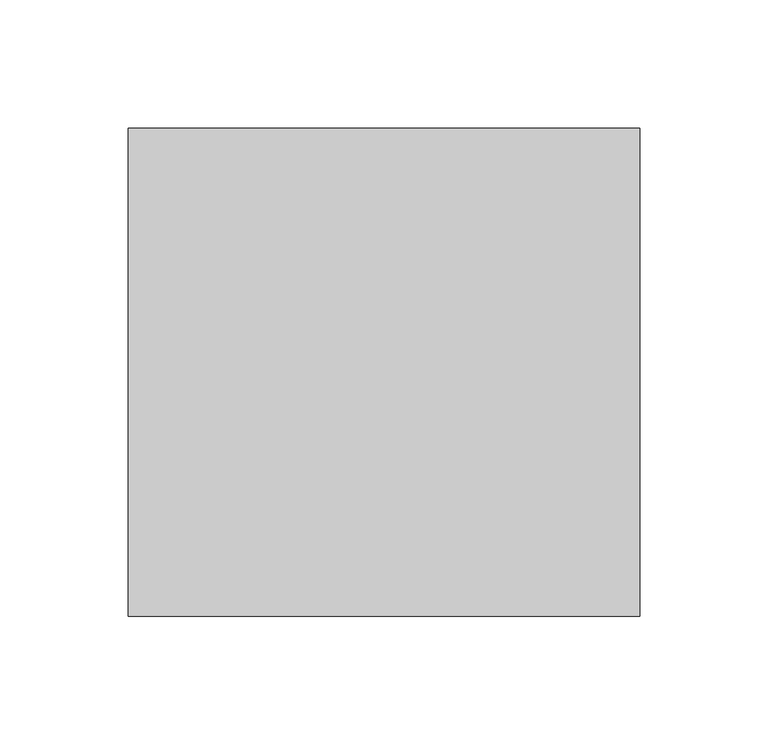
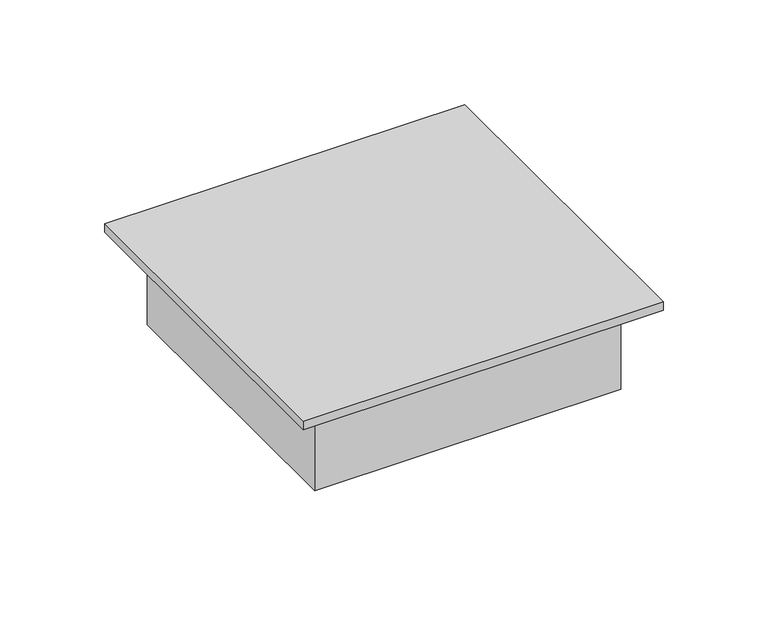
"""IFC4 building model written with IfcOpenShell, lengths in millimetres: proxy geometry, CAIXA VERTICE V7 : QD Amanco Passagem Pequena."""

from ifc_helpers import new_model, si_unit, origin, origin_with_axes, place, context, project, spatial, polyline, outline, extrude, faceted_brep, source, transform, mapped, element, save


def electrical_fixtures_13f3b859(model_context):
    return source(origin(), model_context, "Body", "SolidModel", [
        faceted_brep([(82.5, 1022.0, -48.0), (82.5, 1178.0, -48.0), (-82.5, 1178.0, -48.0), (-82.5, 1022.0, -48.0), (84.5, 1180.0, -50.0), (84.5, 1020.0, -50.0), (-84.5, 1020.0, -50.0), (-84.5, 1180.0, -50.0), (-84.5, 1180.0, 0.0), (84.5, 1180.0, 0.0), (-84.5, 1020.0, 0.0), (84.5, 1020.0, 0.0), (82.5, 1178.0, 0.0), (82.5, 1022.0, 0.0), (-82.5, 1022.0, 0.0), (-82.5, 1178.0, 0.0)], [[[0, 1, 2, 3]], [[4, 5, 6, 7]], [[4, 7, 8, 9]], [[8, 7, 6, 10]], [[10, 6, 5, 11]], [[11, 5, 4, 9]], [[9, 8, 10, 11], [12, 13, 14, 15]], [[13, 12, 1, 0]], [[14, 13, 0, 3]], [[15, 14, 3, 2]], [[12, 15, 2, 1]]]),
        extrude(outline(polyline([(99.5, 1195.0), (99.5, 1005.0), (-99.5, 1005.0), (-99.5, 1195.0), (99.5, 1195.0)])), origin_with_axes(), (0.0, 0.0, 1.0), 5.0),
    ])


if __name__ == "__main__":
    model = new_model("IFC4")
    model_context = context("Model", 3, world=origin())
    ifc_project = project(units=[si_unit("LENGTHUNIT", "METRE", prefix="MILLI")], contexts=[model_context])
    site = spatial("IfcSite", under=ifc_project)
    building = spatial("IfcBuilding", under=site)
    placement = place(None, origin())
    electrical_fixtures_shape = electrical_fixtures_13f3b859(model_context)
    element("IfcBuildingElementProxy", 1, Name="CAIXA VERTICE V7 : QD Amanco Passagem Pequena", ObjectType="CAIXA VERTICE V7 : QD Amanco Passagem Pequena", at=placement, inside=building, context=model_context, shape_type="MappedRepresentation", body=[
        mapped(electrical_fixtures_shape, transform((0.0, 0.0, 0.0), x_axis=(1.0, 0.0, 0.0), y_axis=(0.0, 1.0, 0.0), z_axis=(0.0, 0.0, 1.0))),
    ])
    save(model, "model.ifc")

# Revit data of these elements
# Type "CAIXA VERTICE V7 : QD Amanco Passagem Pequena"
#   URL = "www.facebook.com/verticetreinamentos"
#   SEÇÃO [instance default] = ""
#   Rotação [instance default] = 0.00°
#   LARGURA DA TAMPA = 0.199 m
#   BORDA = 0.03 m
#   ALTURA DE INSTALAÇÃO [instance default] = 1.10 m
#   Distância Anotação [instance default] = 0.0015 m
#   ALTURA DA TAMPA = 0.19 m
#   Vertical [instance default] = yes
#   VER SEÇÃO [instance default] = no
#   SHADE ESQ [instance default] = no
#   SHADE DIR [instance default] = yes
#   HORIZONTAL [instance default] = no
#   ANDAR COM A LEGENDA [instance default] = 0
#   Material Tampa [instance default] = Plástico, branco opaco
#   Caixa = element 1798542
#   Anotação = element 1798539
#   Default Elevation = 0
# Element 1 (IfcBuildingElementProxy, "CAIXA VERTICE V7 : QD Amanco Passagem Pequena")
#   Materials on its faces: "Plástico, branco opaco"
# Materials
#   "Plástico, branco opaco": class "Plástico", colour RGB 120 120 120, transparency 0, Description = "Plastic, generic, opaque white", Cost = 0
